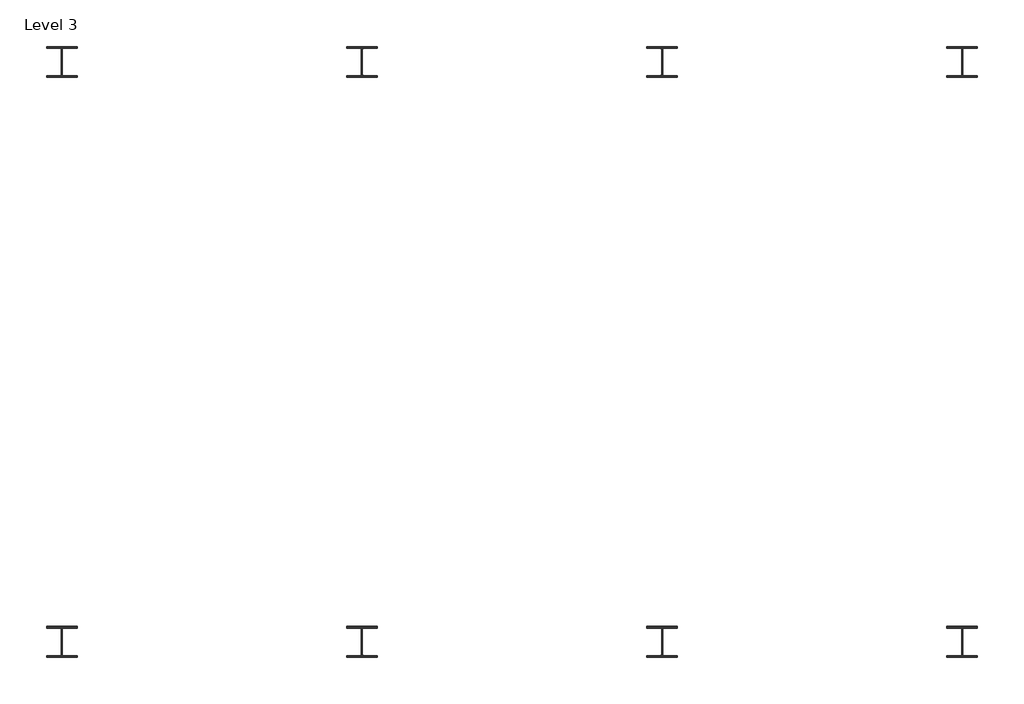
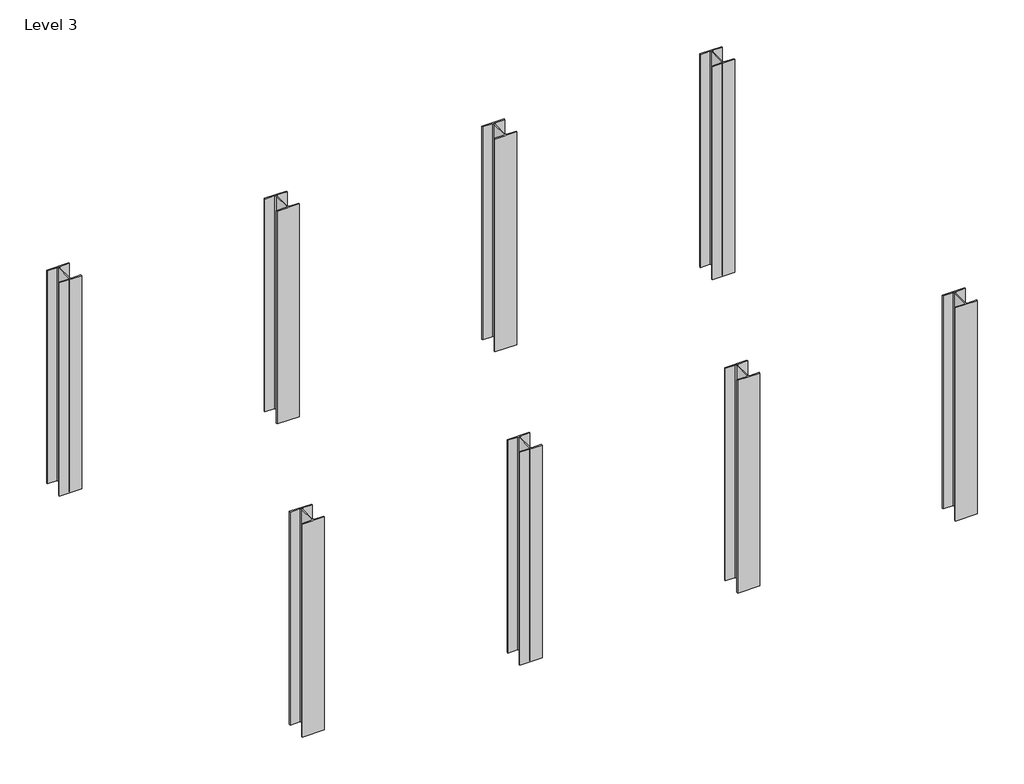
# One storey: 8 columns.
"""IFC4 building model written with IfcOpenShell, lengths in millimetres."""

import ifcopenshell
import ifcopenshell.guid

model = None  # the IFC model being written
_history = None  # IfcOwnerHistory: only IFC2X3 demands one
_inside = {}  # id of a spatial element -> (the spatial element, [elements in it])
_under = {}  # id of a project, library or spatial element -> (it, [spatial elements below it])
_declared = {}  # id of a project -> (the project, [libraries it declares])
_typed = {}  # id of a type object -> (the type object, [elements of that type])
_made_of = {}  # id of a material, layer set ... -> (it, [elements and type objects made of it])


def new_model(schema):
    """Start an empty IFC model of exactly this schema.

    Asked for "IFC4X3", IfcOpenShell would pick the latest addendum, in which some entities
    have other attributes; the version numbers below select the first issue.
    IFC2X3 requires an IfcOwnerHistory on every rooted entity: one is made here for all.
    """
    global model, _history
    if schema == "IFC4X3":
        model = ifcopenshell.file(schema_version=(4, 3, 0, 0))
    else:
        model = ifcopenshell.file(schema=schema)
    _inside.clear()
    _under.clear()
    _declared.clear()
    _typed.clear()
    _made_of.clear()
    _history = None
    if model.schema == "IFC2X3":
        org = make("IfcOrganization", Name="unknown")
        user = make(
            "IfcPersonAndOrganization",
            ThePerson=make("IfcPerson", FamilyName="unknown"),
            TheOrganization=org,
        )
        app = make(
            "IfcApplication",
            ApplicationDeveloper=org,
            Version="unknown",
            ApplicationFullName="unknown",
            ApplicationIdentifier="unknown",
        )
        _history = make(
            "IfcOwnerHistory",
            OwningUser=user,
            OwningApplication=app,
            ChangeAction="ADDED",
            CreationDate=0,
        )
    return model


def make(cls, **values):
    """One entity of the class cls with the attributes given. An attribute that is None is left unset."""
    return model.create_entity(
        cls, **{name: value for name, value in values.items() if value is not None}
    )


def rooted(cls, **values):
    """An entity with a GlobalId (a new one), such as an element, a storey or a relation."""
    return make(cls, GlobalId=ifcopenshell.guid.new(), OwnerHistory=_history, **values)


def si_unit(unit_type, name, prefix=None):
    """IfcSIUnit, for example si_unit("LENGTHUNIT", "METRE", prefix="MILLI")."""
    return make("IfcSIUnit", UnitType=unit_type, Prefix=prefix, Name=name)


def assignment(units):
    """IfcUnitAssignment: the units of a project."""
    return None if units is None else make("IfcUnitAssignment", Units=units)


def point(xyz):
    """IfcCartesianPoint."""
    return None if xyz is None else make("IfcCartesianPoint", Coordinates=xyz)


def direction(xyz):
    """IfcDirection."""
    return None if xyz is None else make("IfcDirection", DirectionRatios=xyz)


def frame(location, z_axis=None, x_axis=None):
    """IfcAxis2Placement3D, a coordinate frame: its origin and axes. An axis left out is left unset."""
    return make(
        "IfcAxis2Placement3D",
        Location=point(location),
        Axis=direction(z_axis),
        RefDirection=direction(x_axis),
    )


def frame_2d(location, x_axis=None):
    """IfcAxis2Placement2D, a coordinate frame in the plane: its origin and x axis."""
    return make(
        "IfcAxis2Placement2D", Location=point(location), RefDirection=direction(x_axis)
    )


def origin():
    """The frame at (0, 0, 0) with its axes left unset."""
    return frame((0.0, 0.0, 0.0))


def place(relative_to, where):
    """IfcLocalPlacement: puts the frame where relative to a parent placement (None: the world)."""
    return make(
        "IfcLocalPlacement", PlacementRelTo=relative_to, RelativePlacement=where
    )


def context(
    kind, dimensions, precision=None, world=None, true_north=None, identifier=None
):
    """IfcGeometricRepresentationContext, for example the 3D "Model" context."""
    return make(
        "IfcGeometricRepresentationContext",
        ContextIdentifier=identifier,
        ContextType=kind,
        CoordinateSpaceDimension=dimensions,
        Precision=precision,
        WorldCoordinateSystem=world,
        TrueNorth=true_north,
    )


def project(units=None, contexts=None):
    """IfcProject with its units and contexts."""
    return rooted(
        "IfcProject",
        Name="project",
        RepresentationContexts=contexts,
        UnitsInContext=assignment(units),
    )


def spatial(cls, under=None, at=None, **own):
    """A site, building, storey or space (cls), placed at a placement, below another one or the project."""
    s = rooted(cls, ObjectPlacement=at, **own)
    if under is not None:
        _under.setdefault(under.id(), (under, []))[1].append(s)
    return s


def polyline(points):
    """IfcPolyline through the points."""
    return make("IfcPolyline", Points=[point(p) for p in points])


def circle_curve(where, radius):
    """IfcCircle in the frame where."""
    return make("IfcCircle", Position=where, Radius=radius)


def trimmed(basis, trim1, trim2, sense, master):
    """IfcTrimmedCurve: the piece of a basis curve between two trims."""
    return make(
        "IfcTrimmedCurve",
        BasisCurve=basis,
        Trim1=trim1,
        Trim2=trim2,
        SenseAgreement=sense,
        MasterRepresentation=master,
    )


def segment(curve, same_sense, transition):
    """IfcCompositeCurveSegment."""
    return make(
        "IfcCompositeCurveSegment",
        Transition=transition,
        SameSense=same_sense,
        ParentCurve=curve,
    )


def composite_curve(segments, self_intersect=None):
    """IfcCompositeCurve: segments joined end to end."""
    return make("IfcCompositeCurve", Segments=segments, SelfIntersect=self_intersect)


def outline(outer, holes=None, kind="AREA"):
    """IfcArbitraryClosedProfileDef: a profile drawn as a closed curve; with holes, ...WithVoids."""
    if holes is None:
        return make("IfcArbitraryClosedProfileDef", ProfileType=kind, OuterCurve=outer)
    return make(
        "IfcArbitraryProfileDefWithVoids",
        ProfileType=kind,
        OuterCurve=outer,
        InnerCurves=holes,
    )


def extrude(swept, where, along, depth):
    """IfcExtrudedAreaSolid: the profile swept, set in the frame where, extruded along a direction by depth."""
    return make(
        "IfcExtrudedAreaSolid",
        SweptArea=swept,
        Position=where,
        ExtrudedDirection=direction(along),
        Depth=depth,
    )


def shape(context_of_items, identifier, shape_type, items):
    """IfcShapeRepresentation: the items that make up one representation, for example the "Body"."""
    return make(
        "IfcShapeRepresentation",
        ContextOfItems=context_of_items,
        RepresentationIdentifier=identifier,
        RepresentationType=shape_type,
        Items=items,
    )


def source(mapping_origin, context_of_items, identifier, shape_type, items):
    """IfcRepresentationMap: a shape defined once, which mapped items show again and again."""
    return make(
        "IfcRepresentationMap",
        MappingOrigin=mapping_origin,
        MappedRepresentation=shape(context_of_items, identifier, shape_type, items),
    )


def transform(
    local_origin,
    x_axis=None,
    y_axis=None,
    z_axis=None,
    scale=None,
    scale2=None,
    scale3=None,
    uniform=True,
):
    """IfcCartesianTransformationOperator3D, or its non-uniform kind. x_axis, y_axis, z_axis: its Axis1, 2, 3."""
    if uniform:
        return make(
            "IfcCartesianTransformationOperator3D",
            Axis1=direction(x_axis),
            Axis2=direction(y_axis),
            LocalOrigin=point(local_origin),
            Scale=scale,
            Axis3=direction(z_axis),
        )
    return make(
        "IfcCartesianTransformationOperator3DnonUniform",
        Axis1=direction(x_axis),
        Axis2=direction(y_axis),
        LocalOrigin=point(local_origin),
        Scale=scale,
        Axis3=direction(z_axis),
        Scale2=scale2,
        Scale3=scale3,
    )


def mapped(mapping_source, mapping_target):
    """IfcMappedItem: shows the shape of a source again, moved by a transform."""
    return make(
        "IfcMappedItem", MappingSource=mapping_source, MappingTarget=mapping_target
    )


def made_of(thing, what):
    """Note that an element or type object is made of a material, layer set ...; save() writes the relation."""
    if what is not None:
        _made_of.setdefault(what.id(), (what, []))[1].append(thing)
    return thing


def element(
    cls,
    number,
    at=None,
    inside=None,
    cuts=None,
    type_object=None,
    material=None,
    context=None,
    identifier="Body",
    shape_type=None,
    held_by="IfcProductDefinitionShape",
    body=None,
    shapes=None,
    **own,
):
    """One element of the class cls, such as IfcWall. Its Tag is "e" and its number.

    at: its placement. inside: the storey or other place that contains it. cuts: it is an
    opening in that element (IfcRelVoidsElement). A single representation is given by context,
    identifier, shape_type and body (its items); several are given by shapes. held_by: the class
    of the entity that holds the representations. save() writes the other relations.
    """
    e = rooted(cls, Tag="e%d" % number, ObjectPlacement=at, **own)
    if body is not None:
        shapes = [shape(context, identifier, shape_type, body)]
    if shapes is not None:
        e.Representation = make(held_by, Representations=shapes)
    if inside is not None:
        _inside.setdefault(inside.id(), (inside, []))[1].append(e)
    if cuts is not None:
        rooted(
            "IfcRelVoidsElement", RelatingBuildingElement=cuts, RelatedOpeningElement=e
        )
    if type_object is not None:
        _typed.setdefault(type_object.id(), (type_object, []))[1].append(e)
    return made_of(e, material)


def aggregate(whole, parts):
    """IfcRelAggregates: a whole, such as a stair, and the parts it consists of."""
    return rooted("IfcRelAggregates", RelatingObject=whole, RelatedObjects=parts)


def save(model, path):
    """Write the relations noted so far, then the file.

    IfcRelAggregates (storeys below a building ...), IfcRelContainedInSpatialStructure (elements
    in a storey), IfcRelDefinesByType, IfcRelAssociatesMaterial and IfcRelDeclares: one each for
    every whole, place, type object, material and project.
    """
    for whole, parts in _under.values():
        aggregate(whole, parts)
    for where, things in _inside.values():
        rooted(
            "IfcRelContainedInSpatialStructure",
            RelatedElements=things,
            RelatingStructure=where,
        )
    for kind, things in _typed.values():
        rooted("IfcRelDefinesByType", RelatedObjects=things, RelatingType=kind)
    for what, things in _made_of.values():
        rooted("IfcRelAssociatesMaterial", RelatedObjects=things, RelatingMaterial=what)
    for by, libraries in _declared.values():
        rooted("IfcRelDeclares", RelatingContext=by, RelatedDefinitions=libraries)
    model.write(path)


def uc_universal_columns_column_uc305x305x97_b067ee91(model_context):
    return source(origin(), model_context, "Body", "SweptSolid", [
        extrude(outline(composite_curve([segment(polyline([(152.65, 153.95), (152.65, 138.55), (20.15, 138.55)]), True, "CONTINUOUS"), segment(trimmed(circle_curve(frame_2d((20.15, 123.35)), 15.2), [point((20.15, 138.55))], [point((4.95, 123.35))], True, "CARTESIAN"), True, "CONTINUOUS"), segment(polyline([(4.95, 123.35), (4.95, -123.35)]), True, "CONTINUOUS"), segment(trimmed(circle_curve(frame_2d((20.15, -123.35)), 15.2), [point((4.95, -123.35))], [point((20.15, -138.55))], True, "CARTESIAN"), True, "CONTINUOUS"), segment(polyline([(20.15, -138.55), (152.65, -138.55), (152.65, -153.95), (-152.65, -153.95), (-152.65, -138.55), (-20.15, -138.55)]), True, "CONTINUOUS"), segment(trimmed(circle_curve(frame_2d((-20.15, -123.35)), 15.2), [point((-20.15, -138.55))], [point((-4.95, -123.35))], True, "CARTESIAN"), True, "CONTINUOUS"), segment(polyline([(-4.95, -123.35), (-4.95, 123.35)]), True, "CONTINUOUS"), segment(trimmed(circle_curve(frame_2d((-20.15, 123.35)), 15.2), [point((-4.95, 123.35))], [point((-20.15, 138.55))], True, "CARTESIAN"), True, "CONTINUOUS"), segment(polyline([(-20.15, 138.55), (-152.65, 138.55), (-152.65, 153.95), (152.65, 153.95)]), True, "CONTINUOUS")], self_intersect=False)), frame((0.0, 0.0, 2900.0), z_axis=(0.0, 0.0, 1.0), x_axis=(1.0, 0.0, 0.0)), (0.0, 0.0, 1.0), 3100.0),
    ])


def uc_universal_columns_column_uc305x305x97_d51453b7(model_context):
    return source(origin(), model_context, "Body", "SweptSolid", [
        extrude(outline(composite_curve([segment(polyline([(152.65, 153.95), (152.65, 138.55), (20.15, 138.55)]), True, "CONTINUOUS"), segment(trimmed(circle_curve(frame_2d((20.15, 123.35)), 15.2), [point((20.15, 138.55))], [point((4.95, 123.35))], True, "CARTESIAN"), True, "CONTINUOUS"), segment(polyline([(4.95, 123.35), (4.95, -123.35)]), True, "CONTINUOUS"), segment(trimmed(circle_curve(frame_2d((20.15, -123.35)), 15.2), [point((4.95, -123.35))], [point((20.15, -138.55))], True, "CARTESIAN"), True, "CONTINUOUS"), segment(polyline([(20.15, -138.55), (152.65, -138.55), (152.65, -153.95), (-152.65, -153.95), (-152.65, -138.55), (-20.15, -138.55)]), True, "CONTINUOUS"), segment(trimmed(circle_curve(frame_2d((-20.15, -123.35)), 15.2), [point((-20.15, -138.55))], [point((-4.95, -123.35))], True, "CARTESIAN"), True, "CONTINUOUS"), segment(polyline([(-4.95, -123.35), (-4.95, 123.35)]), True, "CONTINUOUS"), segment(trimmed(circle_curve(frame_2d((-20.15, 123.35)), 15.2), [point((-4.95, 123.35))], [point((-20.15, 138.55))], True, "CARTESIAN"), True, "CONTINUOUS"), segment(polyline([(-20.15, 138.55), (-152.65, 138.55), (-152.65, 153.95), (152.65, 153.95)]), True, "CONTINUOUS")], self_intersect=False)), frame((0.0, 0.0, 2900.0), z_axis=(0.0, 0.0, 1.0), x_axis=(1.0, 0.0, 0.0)), (0.0, 0.0, 1.0), 3105.0),
    ])


model = new_model("IFC4")

# Units and contexts
model_context = context("Model", 3, world=origin())
ifc_project = project(units=[si_unit("LENGTHUNIT", "METRE", prefix="MILLI")], contexts=[model_context])

# Site, building, storey
site = spatial("IfcSite", under=ifc_project)
building = spatial("IfcBuilding", under=site)
storey = spatial("IfcBuildingStorey", under=building, Name="Level 3", Elevation=3000.0)

# Columns
placement = place(None, origin())
uc_universal_columns_column_uc305x305x97_shape = uc_universal_columns_column_uc305x305x97_b067ee91(model_context)
element("IfcColumn", 1, ObjectType="UC-Universal Columns-Column : UC305x305x97", at=placement, inside=storey, context=model_context, shape_type="MappedRepresentation", body=[
    mapped(uc_universal_columns_column_uc305x305x97_shape, transform((-1938.0684826, 2696.9060214, 0.0), x_axis=(-1.0, 0.0, 0.0), y_axis=(0.0, -1.0, 0.0), z_axis=(0.0, 0.0, 1.0))),
])
element("IfcColumn", 2, ObjectType="UC-Universal Columns-Column : UC305x305x97", at=placement, inside=storey, context=model_context, shape_type="MappedRepresentation", body=[
    mapped(uc_universal_columns_column_uc305x305x97_shape, transform((-1938.0684826, -3100.0939786, 0.0), x_axis=(-1.0, 0.0, 0.0), y_axis=(0.0, -1.0, 0.0), z_axis=(0.0, 0.0, 1.0))),
])
element("IfcColumn", 3, ObjectType="UC-Universal Columns-Column : UC305x305x97", at=placement, inside=storey, context=model_context, shape_type="MappedRepresentation", body=[
    mapped(uc_universal_columns_column_uc305x305x97_shape, transform((1061.9315174, 2696.9060214, 0.0), x_axis=(-1.0, 0.0, 0.0), y_axis=(0.0, -1.0, 0.0), z_axis=(0.0, 0.0, 1.0))),
])
element("IfcColumn", 4, ObjectType="UC-Universal Columns-Column : UC305x305x97", at=placement, inside=storey, context=model_context, shape_type="MappedRepresentation", body=[
    mapped(uc_universal_columns_column_uc305x305x97_shape, transform((1061.9315174, -3100.0939786, 0.0), x_axis=(-1.0, 0.0, 0.0), y_axis=(0.0, -1.0, 0.0), z_axis=(0.0, 0.0, 1.0))),
])
uc_universal_columns_column_uc305x305x97_2_shape = uc_universal_columns_column_uc305x305x97_d51453b7(model_context)
element("IfcColumn", 5, ObjectType="UC-Universal Columns-Column : UC305x305x97", at=placement, inside=storey, context=model_context, shape_type="MappedRepresentation", body=[
    mapped(uc_universal_columns_column_uc305x305x97_2_shape, transform((-4938.0684826, 2696.9060214, 0.0), x_axis=(-1.0, 0.0, 0.0), y_axis=(0.0, -1.0, 0.0), z_axis=(0.0, 0.0, 1.0))),
])
element("IfcColumn", 6, ObjectType="UC-Universal Columns-Column : UC305x305x97", at=placement, inside=storey, context=model_context, shape_type="MappedRepresentation", body=[
    mapped(uc_universal_columns_column_uc305x305x97_2_shape, transform((-4938.0684826, -3100.0939786, 0.0), x_axis=(-1.0, 0.0, 0.0), y_axis=(0.0, -1.0, 0.0), z_axis=(0.0, 0.0, 1.0))),
])
element("IfcColumn", 7, ObjectType="UC-Universal Columns-Column : UC305x305x97", at=placement, inside=storey, context=model_context, shape_type="MappedRepresentation", body=[
    mapped(uc_universal_columns_column_uc305x305x97_2_shape, transform((4061.9315174, 2696.9060214, 0.0), x_axis=(-1.0, 0.0, 0.0), y_axis=(0.0, -1.0, 0.0), z_axis=(0.0, 0.0, 1.0))),
])
element("IfcColumn", 8, ObjectType="UC-Universal Columns-Column : UC305x305x97", at=placement, inside=storey, context=model_context, shape_type="MappedRepresentation", body=[
    mapped(uc_universal_columns_column_uc305x305x97_2_shape, transform((4061.9315174, -3100.0939786, 0.0), x_axis=(-1.0, 0.0, 0.0), y_axis=(0.0, -1.0, 0.0), z_axis=(0.0, 0.0, 1.0))),
])

save(model, "model.ifc")

# Revit data of these elements
# Type "UC-Universal Columns-Column : UC305x305x97"
#   Section Name Key = "UC305x305x97"
#   Cost = 2
#   Width = 30.53 cm
#   Web Thickness = 0.99 cm
#   Web Fillet = 1.52 cm
#   Warping Constant = 1560000.0 cm⁶
#   Torsional Moment of Inertia = 91.20 cm⁴
#   Section Area = 123.0 cm²
#   Plastic Modulus weak axis = 726.0 cm³
#   Plastic Modulus strong axis = 1592.0 cm³
#   Nominal Weight = 96.8996 kgf/m
#   Moment of Inertia weak axis = 7308.00 cm⁴
#   Moment of Inertia strong axis = 22249.00 cm⁴
#   Height = 30.79 cm
#   Flange Thickness = 1.54 cm
#   Elastic Modulus weak axis = 479.0 cm³
#   Elastic Modulus strong axis = 1445.0 cm³
#   Centroid Vertical = 15.395 cm
#   Centroid Horizontal = 15.265 cm
#   Bolt Spacing = 14.0 cm
#   Structural Material [instance default] = Metal - Steel 43-275
#   Type Comments = ""
#   Assembly Code = ""
# Elements 1, 2, 3, 4, 5, 6, 7, 8 (IfcColumn, "UC-Universal Columns-Column : UC305x305x97")
#   Structural Material = Metal - Steel 43-275
#   Phase Created = New Construction
#   Materials on its faces: "Metal - Steel 43-275"
# Materials
#   "Metal - Steel 43-275": class "Metal", colour RGB 247 247 247, transparency 0, Cost = 0
